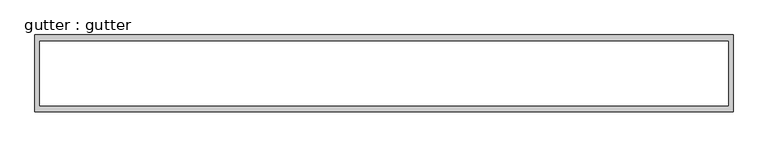
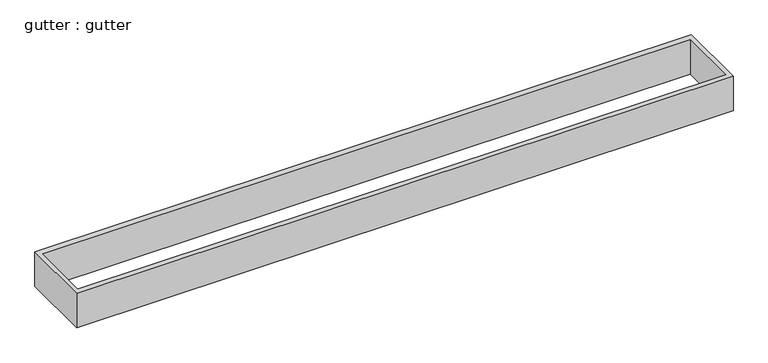
"""IFC4 building model written with IfcOpenShell, lengths in millimetres: proxy geometry, gutter : gutter."""

from ifc_helpers import new_model, si_unit, frame, origin, place, context, project, spatial, polyline, outline, extrude, source, transform, mapped, element, save


def gutter_gutter_dc17c88e(model_context):
    return source(origin(), model_context, "Body", "SweptSolid", [
        extrude(outline(polyline([(23406.8870052, 1909.5502616), (17901.4334333, 1909.5502616), (17901.4334333, 2515.8615366), (23406.8870052, 2515.8615366), (23406.8870052, 1909.5502616)]), holes=[polyline([(23370.1856701, 2465.0615366), (17939.5370052, 2465.0615366), (17939.5370052, 1956.0872459), (23370.1856701, 1956.0872459), (23370.1856701, 2465.0615366)])]), frame((0.0, 0.0, 2832.1), z_axis=(0.0, 0.0, 1.0), x_axis=(1.0, 0.0, 0.0)), (0.0, 0.0, 1.0), 304.8),
    ])


if __name__ == "__main__":
    model = new_model("IFC4")
    model_context = context("Model", 3, world=origin())
    ifc_project = project(units=[si_unit("LENGTHUNIT", "METRE", prefix="MILLI")], contexts=[model_context])
    site = spatial("IfcSite", under=ifc_project)
    building = spatial("IfcBuilding", under=site)
    placement = place(None, origin())
    gutter_gutter_shape = gutter_gutter_dc17c88e(model_context)
    element("IfcBuildingElementProxy", 1, Name="gutter : gutter", ObjectType="gutter : gutter", at=placement, inside=building, context=model_context, shape_type="MappedRepresentation", body=[
        mapped(gutter_gutter_shape, transform((0.0, 0.0, 0.0), x_axis=(1.0, 0.0, 0.0), y_axis=(0.0, 1.0, 0.0), z_axis=(0.0, 0.0, 1.0))),
    ])
    save(model, "model.ifc")
